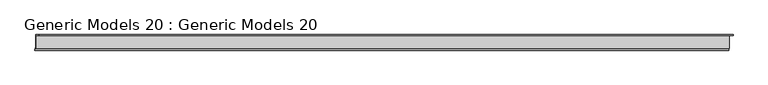
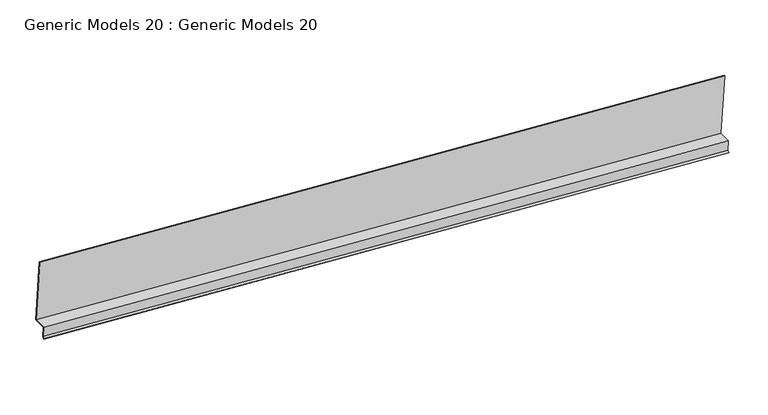
"""IFC4 building model written with IfcOpenShell, lengths in millimetres: proxy geometry, Generic Models 20 : Generic Models 20."""

from ifc_helpers import new_model, si_unit, frame, origin, place, context, project, spatial, polyline, outline, extrude, source, transform, mapped, element, save


def generic_models_20_generic_models_20_568b0388(model_context):
    return source(origin(), model_context, "Body", "SweptSolid", [
        extrude(outline(polyline([(0.0, 0.0), (0.0, -131.7625), (-1.5875, -131.7625), (-1.5875, -1.5875), (-30.1625, -1.5875), (-30.1625, 19.3223719), (-33.7226921, 22.8825641), (-32.6001601, 24.005096), (-28.575, 19.979936), (-28.575, 0.0), (0.0, 0.0)])), frame((28940.214405, 25528.2178246, 272576.0987961), z_axis=(-0.9980525759468354, 0.0, 0.06237832673201991), x_axis=(0.0, 1.0, 0.0)), (0.0, 0.0, 1.0), 1498.6),
    ])


if __name__ == "__main__":
    model = new_model("IFC4")
    model_context = context("Model", 3, world=origin())
    ifc_project = project(units=[si_unit("LENGTHUNIT", "METRE", prefix="MILLI")], contexts=[model_context])
    site = spatial("IfcSite", under=ifc_project)
    building = spatial("IfcBuilding", under=site)
    placement = place(None, origin())
    generic_models_20_generic_models_20_shape = generic_models_20_generic_models_20_568b0388(model_context)
    element("IfcBuildingElementProxy", 1, Name="Generic Models 20 : Generic Models 20", ObjectType="Generic Models 20 : Generic Models 20", at=placement, inside=building, context=model_context, shape_type="MappedRepresentation", body=[
        mapped(generic_models_20_generic_models_20_shape, transform((0.0, 0.0, 0.0), x_axis=(1.0, 0.0, 0.0), y_axis=(0.0, 1.0, 0.0), z_axis=(0.0, 0.0, 1.0))),
    ])
    save(model, "model.ifc")

# Revit data of these elements
# Element 1 (IfcBuildingElementProxy, "Generic Models 20 : Generic Models 20")
#   Materials on its faces: "SEAMLESS CONCEALED SHEET METAL GUTTER - (COLOR: EXTRA DARK BRONZE)"
# Materials
#   "SEAMLESS CONCEALED SHEET METAL GUTTER - (COLOR: EXTRA DARK BRONZE)": class "Generic", colour RGB 97 74 67, transparency 0, Cost = 0
